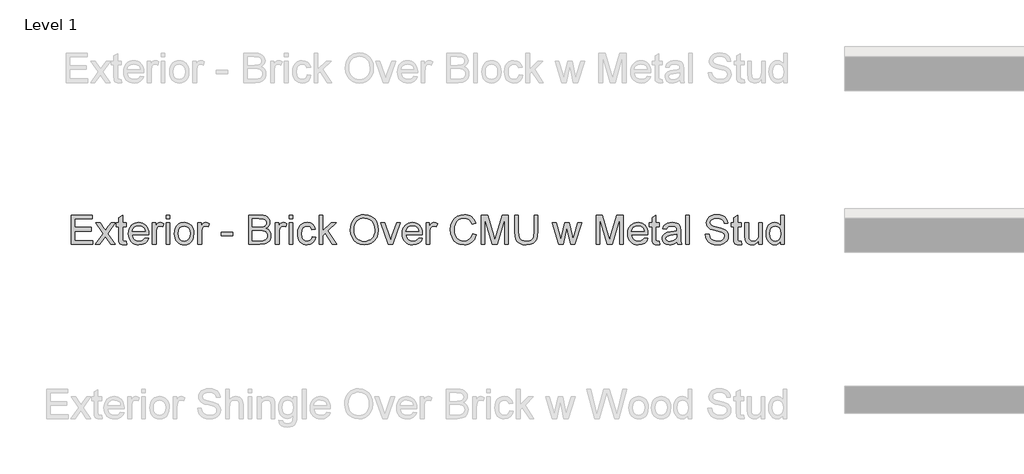
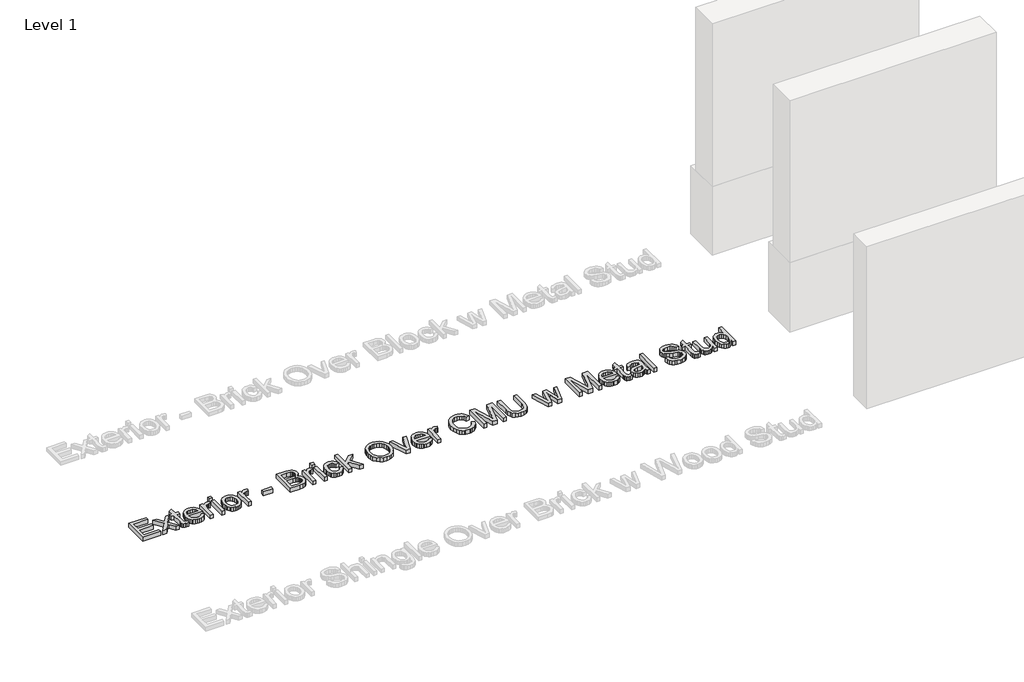
# One storey, part 39 of 42: 1 proxy.
"""IFC4 building model written with IfcOpenShell, lengths in millimetres."""

from ifc_helpers import new_model, si_unit, origin, origin_with_axes, place, context, project, spatial, polyline, outline, extrude, element, save

model = new_model("IFC4")

# Units and contexts
model_context = context("Model", 3, world=origin())
ifc_project = project(units=[si_unit("LENGTHUNIT", "METRE", prefix="MILLI")], contexts=[model_context])

# Site, building, storey
site = spatial("IfcSite", under=ifc_project)
building = spatial("IfcBuilding", under=site)
storey = spatial("IfcBuildingStorey", under=building, Name="Level 1", Elevation=0.0)

# Proxy
placement = place(None, origin())
element("IfcBuildingElementProxy", 1, Name="8\" Arial", ObjectType="8\" Arial", at=placement, inside=storey, context=model_context, shape_type="SweptSolid", body=[
    extrude(outline(polyline([(27482.7881133, 15014.0462247), (27482.7881133, 15318.6133187), (27701.6957121, 15318.6133187), (27701.6957121, 15280.542432), (27520.859, 15280.542432), (27520.859, 15190.1240759), (27692.1779905, 15190.1240759), (27692.1779905, 15152.0531892), (27520.859, 15152.0531892), (27520.859, 15052.1171114), (27706.454573, 15052.1171114), (27706.454573, 15014.0462247), (27482.7881133, 15014.0462247)])), origin_with_axes(), (0.0, 0.0, 1.0), 50.8),
    extrude(outline(polyline([(27735.0077381, 15014.0462247), (27816.3545156, 15126.4743121), (27739.7665989, 15237.7126844), (27785.5706345, 15237.7126844), (27822.5261633, 15184.1754999), (27839.7770338, 15158.8940516), (27854.7228312, 15179.5653534), (27896.8090068, 15237.7126844), (27942.6130424, 15237.7126844), (27862.1585513, 15126.4743121), (27939.6387544, 15014.0462247), (27893.8347188, 15014.0462247), (27847.2127539, 15081.6369201), (27838.6616758, 15093.9802154), (27780.8117737, 15014.0462247), (27735.0077381, 15014.0462247)])), origin_with_axes(), (0.0, 0.0, 1.0), 50.8),
    extrude(outline(polyline([(28053.8514147, 15045.7967494), (28058.6102755, 15012.9308667), (28030.1314676, 15009.2873638), (28011.8581856, 15010.8674543), (27998.2322285, 15015.6077259), (27988.602971, 15022.9133208), (27982.3197876, 15032.1893816), (27978.8621778, 15048.1204119), (27977.7096411, 15075.3909152), (27977.7096411, 15199.6417976), (27949.1564761, 15199.6417976), (27949.1564761, 15237.7126844), (27977.7096411, 15237.7126844), (27977.7096411, 15292.0677981), (28015.7805279, 15314.4493155), (28015.7805279, 15237.7126844), (28053.8514147, 15237.7126844), (28053.8514147, 15199.6417976), (28015.7805279, 15199.6417976), (28015.7805279, 15076.5062732), (28017.7881723, 15056.8759723), (28024.2944274, 15049.923574), (28037.2697589, 15047.3582506), (28053.8514147, 15045.7967494)])), origin_with_axes(), (0.0, 0.0, 1.0), 50.8),
    extrude(outline(polyline([(28248.5185661, 15080.6702765), (28285.8458808, 15075.9114156), (28272.3965222, 15047.7858045), (28250.9351751, 15026.761306), (28221.9451615, 15013.6558494), (28185.9098031, 15009.2873638), (28162.2874499, 15011.1718541), (28141.2397148, 15016.825325), (28122.7665977, 15026.2477766), (28106.8680988, 15039.4392087), (28094.0833076, 15056.0324828), (28084.9513139, 15075.6604601), (28079.4721176, 15098.3231407), (28077.6457189, 15124.0205245), (28079.4907069, 15150.5892818), (28085.0256711, 15174.0071527), (28094.2506113, 15194.2741372), (28107.1655276, 15211.3902353), (28123.0222006, 15224.9883084), (28141.0724111, 15234.7012177), (28161.316159, 15240.5289633), (28183.7534443, 15242.4715452), (28205.4680706, 15240.5336107), (28225.1053425, 15234.719807), (28242.6652602, 15225.0301343), (28258.1478236, 15211.4645925), (28270.786224, 15194.385673), (28279.8136529, 15174.1558671), (28285.2301103, 15150.7751748), (28287.0355961, 15124.2435961), (28286.8125245, 15113.9823024), (28115.7166056, 15113.9823024), (28122.3065126, 15085.4849052), (28137.6148013, 15064.5347639), (28159.7081845, 15051.6523789), (28186.6533751, 15047.3582506), (28206.9157123, 15049.3473057), (28223.9806899, 15055.3144711), (28237.8483078, 15065.6315326), (28248.5185661, 15080.6702765)]), holes=[polyline([(28115.7166056, 15152.0531892), (28248.9647093, 15152.0531892), (28243.8154732, 15172.166812), (28233.7214832, 15186.5549303), (28211.5258587, 15199.9392264), (28183.6047299, 15204.4006585), (28157.942201, 15200.8408075), (28136.7225148, 15190.1612545), (28121.9719052, 15173.5145362), (28115.7166056, 15152.0531892)])]), origin_with_axes(), (0.0, 0.0, 1.0), 50.8),
    extrude(outline(polyline([(28325.1064828, 15014.0462247), (28325.1064828, 15237.7126844), (28358.4185087, 15237.7126844), (28358.4185087, 15204.6237301), (28370.7246254, 15223.8078878), (28382.0640986, 15235.1101823), (28393.4407503, 15240.6312045), (28405.8584028, 15242.4715452), (28424.819489, 15239.5344358), (28444.0780039, 15230.7231075), (28431.3629226, 15196.5931524), (28417.9786265, 15202.4487819), (28404.5943304, 15204.4006585), (28393.2269733, 15202.5231391), (28383.0679208, 15196.8905812), (28374.8607447, 15187.9305385), (28369.3490172, 15176.070565), (28364.7202815, 15154.8044056), (28363.1773696, 15131.604959), (28363.1773696, 15014.0462247), (28325.1064828, 15014.0462247)])), origin_with_axes(), (0.0, 0.0, 1.0), 50.8),
    extrude(outline(polyline([(28467.8723082, 15280.542432), (28467.8723082, 15318.6133187), (28505.9431949, 15318.6133187), (28505.9431949, 15280.542432), (28467.8723082, 15280.542432)])), origin_with_axes(), (0.0, 0.0, 1.0), 50.8),
    extrude(outline(polyline([(28467.8723082, 15014.0462247), (28467.8723082, 15237.7126844), (28505.9431949, 15237.7126844), (28505.9431949, 15014.0462247), (28467.8723082, 15014.0462247)])), origin_with_axes(), (0.0, 0.0, 1.0), 50.8),
    extrude(outline(polyline([(28553.5318034, 15125.8794545), (28555.5905684, 15154.8462315), (28561.7668633, 15179.8070143), (28572.0606883, 15200.7618029), (28586.4720433, 15217.7105974), (28600.9809921, 15228.5435121), (28616.9956742, 15236.2813083), (28634.5160896, 15240.923986), (28653.5422383, 15242.4715452), (28674.5458238, 15240.5870549), (28693.5371176, 15234.933584), (28710.5161197, 15225.5111325), (28725.48283, 15212.3197003), (28737.6983239, 15195.8054308), (28746.4236766, 15176.414467), (28751.6588883, 15154.1468091), (28753.4039589, 15129.0024569), (28750.318135, 15090.5411949), (28741.0606635, 15061.2630471), (28725.9010892, 15039.3369675), (28705.108957, 15022.9319101), (28680.4130717, 15012.6985004), (28653.5422383, 15009.2873638), (28632.2319293, 15011.1648831), (28613.0640372, 15016.7974411), (28596.0385619, 15026.1850377), (28581.1555034, 15039.3276729), (28569.0701347, 15056.0022752), (28560.4377284, 15075.9857728), (28555.2582846, 15099.278166), (28553.5318034, 15125.8794545)]), holes=[polyline([(28591.6026901, 15125.9538117), (28596.0083543, 15091.4985438), (28609.2253467, 15066.951373), (28629.1158979, 15052.2565312), (28653.5422383, 15047.3582506), (28677.8570429, 15052.2844151), (28697.7104155, 15067.0629088), (28710.927408, 15091.9353924), (28715.3330721, 15127.1435269), (28710.899524, 15160.5949726), (28697.5988797, 15184.8075361), (28677.7176232, 15199.5023779), (28653.5422383, 15204.4006585), (28629.1158979, 15199.5209672), (28609.2253467, 15184.8818933), (28596.0083543, 15160.3904903), (28591.6026901, 15125.9538117)])]), origin_with_axes(), (0.0, 0.0, 1.0), 50.8),
    extrude(outline(polyline([(28796.2337065, 15014.0462247), (28796.2337065, 15237.7126844), (28829.5457324, 15237.7126844), (28829.5457324, 15204.6237301), (28841.8518491, 15223.8078878), (28853.1913222, 15235.1101823), (28864.5679739, 15240.6312045), (28876.9856264, 15242.4715452), (28895.9467126, 15239.5344358), (28915.2052276, 15230.7231075), (28902.4901463, 15196.5931524), (28889.1058501, 15202.4487819), (28875.721554, 15204.4006585), (28864.3541969, 15202.5231391), (28854.1951444, 15196.8905812), (28845.9879684, 15187.9305385), (28840.4762409, 15176.070565), (28835.8475051, 15154.8044056), (28834.3045932, 15131.604959), (28834.3045932, 15014.0462247), (28796.2337065, 15014.0462247)])), origin_with_axes(), (0.0, 0.0, 1.0), 50.8),
    extrude(outline(polyline([(29038.9356095, 15104.4645807), (29038.9356095, 15142.5354675), (29157.9071307, 15142.5354675), (29157.9071307, 15104.4645807), (29038.9356095, 15104.4645807)])), origin_with_axes(), (0.0, 0.0, 1.0), 50.8),
    extrude(outline(polyline([(29324.4672602, 15014.0462247), (29324.4672602, 15318.6133187), (29440.6875649, 15318.6133187), (29472.6518666, 15316.3733081), (29497.6080021, 15309.653276), (29516.7363919, 15298.285919), (29531.2174568, 15282.1039332), (29540.3355085, 15263.0684898), (29543.3748591, 15243.14076), (29540.8188303, 15224.8024154), (29533.150744, 15207.5608395), (29520.3148322, 15192.4756224), (29502.2553271, 15180.6063542), (29523.82821, 15169.3412383), (29539.7685349, 15152.2019036), (29549.6115693, 15130.3222973), (29552.8925808, 15104.8363667), (29550.6525701, 15083.5980913), (29543.9325381, 15063.9027277), (29533.9036107, 15047.1537683), (29521.7369137, 15034.7547051), (29506.8375896, 15025.7760731), (29488.6107808, 15019.2884073), (29439.7952785, 15014.0462247), (29324.4672602, 15014.0462247)]), holes=[polyline([(29362.538147, 15194.8829368), (29432.0621296, 15194.8829368), (29472.6611612, 15198.1546536), (29486.8726812, 15203.7965062), (29497.0875017, 15212.2453431), (29503.2498547, 15223.3710393), (29505.3039723, 15237.0434696), (29503.3892744, 15250.3162299), (29497.6451807, 15261.8787746), (29488.3319413, 15270.9038798), (29475.7098065, 15276.5643217), (29426.7827684, 15280.542432), (29362.538147, 15280.542432), (29362.538147, 15194.8829368)]), polyline([(29362.538147, 15052.1171114), (29440.6132077, 15052.1171114), (29468.868944, 15053.6042554), (29492.774784, 15061.8950833), (29508.6128678, 15078.8113465), (29513.2694875, 15090.7642665), (29514.821694, 15104.4645807), (29512.9999426, 15120.3770217), (29507.5346884, 15134.0587466), (29497.9890827, 15144.7568888), (29483.9262771, 15151.7185818), (29464.007842, 15155.5386829), (29436.8953477, 15156.81205), (29362.538147, 15156.81205), (29362.538147, 15052.1171114)])]), origin_with_axes(), (0.0, 0.0, 1.0), 50.8),
    extrude(outline(polyline([(29600.4811892, 15014.0462247), (29600.4811892, 15237.7126844), (29633.7932151, 15237.7126844), (29633.7932151, 15204.6237301), (29646.0993319, 15223.8078878), (29657.438805, 15235.1101823), (29668.8154567, 15240.6312045), (29681.2331092, 15242.4715452), (29700.1941954, 15239.5344358), (29719.4527104, 15230.7231075), (29706.737629, 15196.5931524), (29693.3533329, 15202.4487819), (29679.9690368, 15204.4006585), (29668.6016797, 15202.5231391), (29658.4426272, 15196.8905812), (29650.2354511, 15187.9305385), (29644.7237236, 15176.070565), (29640.0949879, 15154.8044056), (29638.552076, 15131.604959), (29638.552076, 15014.0462247), (29600.4811892, 15014.0462247)])), origin_with_axes(), (0.0, 0.0, 1.0), 50.8),
    extrude(outline(polyline([(29743.2470146, 15014.0462247), (29743.2470146, 15237.7126844), (29781.3179013, 15237.7126844), (29781.3179013, 15014.0462247), (29743.2470146, 15014.0462247)])), origin_with_axes(), (0.0, 0.0, 1.0), 50.8),
    extrude(outline(polyline([(29743.2470146, 15280.542432), (29743.2470146, 15318.6133187), (29781.3179013, 15318.6133187), (29781.3179013, 15280.542432), (29743.2470146, 15280.542432)])), origin_with_axes(), (0.0, 0.0, 1.0), 50.8),
    extrude(outline(polyline([(29981.1900568, 15094.946859), (30019.2609436, 15090.1879982), (30008.6464532, 15056.3275879), (29988.7001341, 15030.7394162), (29961.2995056, 15014.6503769), (29928.3220871, 15009.2873638), (29906.9699522, 15011.1579121), (29887.8252967, 15016.7695571), (29870.8881206, 15026.1222988), (29856.1584238, 15039.2161371), (29844.2357114, 15055.8047638), (29835.7194883, 15075.6418708), (29830.6097544, 15098.7274579), (29828.9065098, 15125.0615253), (29831.8157353, 15158.9405249), (29840.5434117, 15188.3023245), (29855.2289588, 15212.0129769), (29876.0117964, 15228.9385347), (29900.8749854, 15239.0882926), (29927.8015867, 15242.4715452), (29959.9703707, 15237.8242202), (29985.6886675, 15223.882245), (30004.1385479, 15201.3891918), (30014.5020827, 15171.0886325), (29976.431196, 15166.3297717), (29969.525271, 15182.9393114), (29958.7713608, 15194.8457582), (29944.7643231, 15202.0119334), (29928.0990155, 15204.4006585), (29903.4960767, 15199.6975655), (29883.9680169, 15185.5882867), (29871.2250516, 15161.3106606), (29866.9773965, 15126.1025261), (29871.1321051, 15090.4203644), (29883.5962309, 15066.0590866), (29902.771094, 15052.0334596), (29927.0580147, 15047.3582506), (29946.7719675, 15050.2767707), (29962.935364, 15059.0323311), (29974.6930964, 15073.8480033), (29981.1900568, 15094.946859)])), origin_with_axes(), (0.0, 0.0, 1.0), 50.8),
    extrude(outline(polyline([(30052.5729695, 15014.0462247), (30052.5729695, 15318.6133187), (30090.6438562, 15318.6133187), (30090.6438562, 15154.95312), (30176.0059227, 15237.7126844), (30228.6508207, 15237.7126844), (30142.2477535, 15153.9121192), (30233.4096816, 15014.0462247), (30188.9440756, 15014.0462247), (30114.9586609, 15127.4409557), (30090.6438562, 15103.8697231), (30090.6438562, 15014.0462247), (30052.5729695, 15014.0462247)])), origin_with_axes(), (0.0, 0.0, 1.0), 50.8),
    extrude(outline(polyline([(30376.1755069, 15162.3144829), (30378.7129464, 15198.0384705), (30386.3252648, 15229.6635174), (30399.0124622, 15257.1896236), (30416.7745385, 15280.6167892), (30438.5472563, 15299.3222725), (30463.2663783, 15312.683332), (30490.9319042, 15320.6999677), (30521.5438343, 15323.3721796), (30561.4922404, 15318.3530685), (30597.3138218, 15303.2957354), (30627.0567021, 15279.2597703), (30648.7690047, 15247.3047633), (30662.041765, 15208.9736263), (30666.4660185, 15165.8092713), (30661.8093988, 15122.068648), (30647.8395397, 15083.1984213), (30625.3278972, 15051.1876464), (30595.0459272, 15028.0253784), (30559.5310692, 15013.9718675), (30521.3207627, 15009.2873638), (30480.7589097, 15014.4644839), (30444.732846, 15029.9958442), (30415.0643229, 15054.4779525), (30393.5750919, 15086.5073167), (30380.5254032, 15123.3606043), (30376.1755069, 15162.3144829)]), holes=[polyline([(30414.2463937, 15161.9426969), (30416.1494733, 15136.7030745), (30421.8587121, 15114.2983205), (30431.3741101, 15094.7284347), (30444.6956674, 15077.9934173), (30460.8892715, 15064.5905318), (30479.0208102, 15055.0170422), (30499.0902834, 15049.2729485), (30521.0976911, 15047.3582506), (30543.4815322, 15049.2915378), (30563.788019, 15055.0913994), (30582.0171514, 15064.7578355), (30598.1689296, 15078.2908461), (30611.392893, 15095.3790603), (30620.8385812, 15115.7111073), (30626.5059941, 15139.2869873), (30628.3951317, 15166.1067001), (30625.1605935, 15199.8091013), (30615.4569788, 15228.9385347), (30599.5352432, 15252.7607229), (30577.6463422, 15270.5413885), (30551.2402413, 15281.6113167), (30521.7669059, 15285.3012928), (30500.5239831, 15283.523691), (30480.8146776, 15278.1908855), (30462.6389894, 15269.3028764), (30445.9969184, 15256.8596635), (30432.1060638, 15240.2617422), (30422.1840249, 15218.9096072), (30416.2308015, 15192.8032588), (30414.2463937, 15161.9426969)])]), origin_with_axes(), (0.0, 0.0, 1.0), 50.8),
    extrude(outline(polyline([(30768.930241, 15014.0462247), (30690.2603227, 15237.7126844), (30730.5619255, 15237.7126844), (30778.2248911, 15103.7210087), (30792.5758309, 15058.6605451), (30806.6293418, 15101.1928639), (30854.5897362, 15237.7126844), (30894.891339, 15237.7126844), (30817.1880643, 15014.0462247), (30768.930241, 15014.0462247)])), origin_with_axes(), (0.0, 0.0, 1.0), 50.8),
    extrude(outline(polyline([(31084.7996296, 15080.6702765), (31122.1269444, 15075.9114156), (31108.6775857, 15047.7858045), (31087.2162386, 15026.761306), (31058.226225, 15013.6558494), (31022.1908666, 15009.2873638), (30998.5685134, 15011.1718541), (30977.5207783, 15016.825325), (30959.0476612, 15026.2477766), (30943.1491623, 15039.4392087), (30930.3643711, 15056.0324828), (30921.2323774, 15075.6604601), (30915.7531811, 15098.3231407), (30913.9267824, 15124.0205245), (30915.7717704, 15150.5892818), (30921.3067346, 15174.0071527), (30930.5316748, 15194.2741372), (30943.4465911, 15211.3902353), (30959.3032641, 15224.9883084), (30977.3534746, 15234.7012177), (30997.5972225, 15240.5289633), (31020.0345078, 15242.4715452), (31041.7491341, 15240.5336107), (31061.386406, 15234.719807), (31078.9463237, 15225.0301343), (31094.4288871, 15211.4645925), (31107.0672876, 15194.385673), (31116.0947165, 15174.1558671), (31121.5111738, 15150.7751748), (31123.3166596, 15124.2435961), (31123.093588, 15113.9823024), (30951.9976692, 15113.9823024), (30958.5875761, 15085.4849052), (30973.8958648, 15064.5347639), (30995.989248, 15051.6523789), (31022.9344386, 15047.3582506), (31043.1967758, 15049.3473057), (31060.2617534, 15055.3144711), (31074.1293713, 15065.6315326), (31084.7996296, 15080.6702765)]), holes=[polyline([(30951.9976692, 15152.0531892), (31085.2457728, 15152.0531892), (31080.0965367, 15172.166812), (31070.0025467, 15186.5549303), (31047.8069223, 15199.9392264), (31019.8857934, 15204.4006585), (30994.2232645, 15200.8408075), (30973.0035784, 15190.1612545), (30958.2529687, 15173.5145362), (30951.9976692, 15152.0531892)])]), origin_with_axes(), (0.0, 0.0, 1.0), 50.8),
    extrude(outline(polyline([(31161.3875463, 15014.0462247), (31161.3875463, 15237.7126844), (31194.6995722, 15237.7126844), (31194.6995722, 15204.6237301), (31207.005689, 15223.8078878), (31218.3451621, 15235.1101823), (31229.7218138, 15240.6312045), (31242.1394663, 15242.4715452), (31261.1005525, 15239.5344358), (31280.3590675, 15230.7231075), (31267.6439861, 15196.5931524), (31254.25969, 15202.4487819), (31240.8753939, 15204.4006585), (31229.5080368, 15202.5231391), (31219.3489843, 15196.8905812), (31211.1418082, 15187.9305385), (31205.6300807, 15176.070565), (31201.001345, 15154.8044056), (31199.4584331, 15131.604959), (31199.4584331, 15014.0462247), (31161.3875463, 15014.0462247)])), origin_with_axes(), (0.0, 0.0, 1.0), 50.8),
    extrude(outline(polyline([(31642.0324917, 15122.3103089), (31680.1033784, 15112.4951584), (31672.5700645, 15088.819361), (31662.5364897, 15068.1317935), (31650.0026541, 15050.4324561), (31634.9685576, 15035.7213487), (31617.7734549, 15024.1564803), (31598.7566008, 15015.89586), (31577.9179954, 15010.9394879), (31555.2576384, 15009.2873638), (31511.0987559, 15014.2878856), (31492.4281275, 15020.5385377), (31476.0300411, 15029.2894508), (31449.149913, 15053.7715591), (31429.5567907, 15087.2137102), (31417.594576, 15126.53008), (31413.6071711, 15168.6348449), (31418.1150764, 15213.044683), (31431.6387923, 15251.3944093), (31453.4719253, 15282.4664245), (31482.9080822, 15305.0431296), (31517.8187879, 15318.7899171), (31556.0755676, 15323.3721796), (31577.8506091, 15321.8896829), (31597.8178412, 15317.4421928), (31615.9772638, 15310.0297094), (31632.328877, 15299.6522326), (31646.6031358, 15286.5839545), (31658.5304956, 15271.0990675), (31675.3445176, 15232.8794663), (31637.2736308, 15223.8078878), (31624.0752277, 15251.5710076), (31606.0436065, 15270.6157457), (31582.9556957, 15281.629906), (31554.5884236, 15285.3012928), (31521.8898446, 15281.2302361), (31495.0283059, 15269.0170659), (31474.6451382, 15249.9444439), (31461.3816726, 15225.2950319), (31454.1039615, 15197.4296709), (31451.6780579, 15168.7092021), (31454.5501047, 15133.5382462), (31463.1662454, 15103.1261511), (31477.8517925, 15078.6347481), (31498.9320589, 15061.2258685), (31524.2042125, 15050.8251551), (31551.4654212, 15047.3582506), (31583.2438299, 15052.0799328), (31609.724288, 15066.2449796), (31629.7170803, 15089.7046764), (31642.0324917, 15122.3103089)])), origin_with_axes(), (0.0, 0.0, 1.0), 50.8),
    extrude(outline(polyline([(31732.4508477, 15014.0462247), (31732.4508477, 15318.6133187), (31797.9595415, 15318.6133187), (31860.2708757, 15103.9440803), (31872.8372426, 15059.1066883), (31886.4446104, 15107.6619403), (31947.7149437, 15318.6133187), (32013.2236376, 15318.6133187), (32013.2236376, 15014.0462247), (31975.1527508, 15014.0462247), (31975.1527508, 15280.542432), (31898.6391913, 15014.0462247), (31847.035294, 15014.0462247), (31770.5217345, 15280.542432), (31770.5217345, 15014.0462247), (31732.4508477, 15014.0462247)])), origin_with_axes(), (0.0, 0.0, 1.0), 50.8),
    extrude(outline(polyline([(32279.7198449, 15318.6133187), (32317.7907316, 15318.6133187), (32317.7907316, 15142.9072535), (32315.2068189, 15101.7598375), (32307.4550807, 15070.0743754), (32292.9740159, 15045.6294457), (32270.2021232, 15026.203627), (32239.0836347, 15013.5164296), (32199.5627825, 15009.2873638), (32160.9063328, 15012.9680453), (32130.0016213, 15024.0100896), (32106.8393532, 15042.0324161), (32091.4102341, 15066.6539442), (32082.7383256, 15099.6778359), (32079.8476894, 15142.9072535), (32079.8476894, 15318.6133187), (32117.9185761, 15318.6133187), (32117.9185761, 15144.2456831), (32119.7960955, 15110.0320761), (32125.4286534, 15086.2098879), (32135.6341792, 15069.711884), (32151.2306021, 15057.4708299), (32171.5672964, 15049.8863954), (32195.9936369, 15047.3582506), (32234.7151491, 15052.3587723), (32249.2101559, 15058.6094245), (32260.4613299, 15067.3603376), (32268.8869302, 15079.6664543), (32274.9052161, 15096.5827174), (32279.7198449, 15144.2456831), (32279.7198449, 15318.6133187)])), origin_with_axes(), (0.0, 0.0, 1.0), 50.8),
    extrude(outline(polyline([(32535.7316869, 15014.0462247), (32467.6948482, 15237.7126844), (32507.252879, 15237.7126844), (32545.8442662, 15107.2157971), (32557.3696323, 15060.5938323), (32566.8129968, 15105.5055815), (32597.5225207, 15237.7126844), (32642.8804131, 15237.7126844), (32673.4412226, 15105.8773675), (32681.8435862, 15065.2039787), (32693.8894528, 15108.1080835), (32732.5551971, 15237.7126844), (32772.2619423, 15237.7126844), (32703.7046033, 15014.0462247), (32657.677496, 15014.0462247), (32628.4551161, 15145.2123267), (32619.9783953, 15186.1087871), (32582.2792945, 15014.0462247), (32535.7316869, 15014.0462247)])), origin_with_axes(), (0.0, 0.0, 1.0), 50.8),
    extrude(outline(polyline([(32922.1660589, 15014.0462247), (32922.1660589, 15318.6133187), (32987.6747527, 15318.6133187), (33049.9860869, 15103.9440803), (33062.5524538, 15059.1066883), (33076.1598216, 15107.6619403), (33137.4301549, 15318.6133187), (33202.9388488, 15318.6133187), (33202.9388488, 15014.0462247), (33164.867962, 15014.0462247), (33164.867962, 15280.542432), (33088.3544025, 15014.0462247), (33036.7505052, 15014.0462247), (32960.2369457, 15280.542432), (32960.2369457, 15014.0462247), (32922.1660589, 15014.0462247)])), origin_with_axes(), (0.0, 0.0, 1.0), 50.8),
    extrude(outline(polyline([(33421.4003044, 15080.6702765), (33458.7276192, 15075.9114156), (33445.2782605, 15047.7858045), (33423.8169134, 15026.761306), (33394.8268998, 15013.6558494), (33358.7915414, 15009.2873638), (33335.1691882, 15011.1718541), (33314.1214531, 15016.825325), (33295.6483361, 15026.2477766), (33279.7498371, 15039.4392087), (33266.9650459, 15056.0324828), (33257.8330522, 15075.6604601), (33252.3538559, 15098.3231407), (33250.5274572, 15124.0205245), (33252.3724452, 15150.5892818), (33257.9074094, 15174.0071527), (33267.1323496, 15194.2741372), (33280.0472659, 15211.3902353), (33295.9039389, 15224.9883084), (33313.9541494, 15234.7012177), (33334.1978973, 15240.5289633), (33356.6351826, 15242.4715452), (33378.3498089, 15240.5336107), (33397.9870808, 15234.719807), (33415.5469985, 15225.0301343), (33431.0295619, 15211.4645925), (33443.6679624, 15194.385673), (33452.6953913, 15174.1558671), (33458.1118486, 15150.7751748), (33459.9173344, 15124.2435961), (33459.6942628, 15113.9823024), (33288.598344, 15113.9823024), (33295.1882509, 15085.4849052), (33310.4965396, 15064.5347639), (33332.5899228, 15051.6523789), (33359.5351134, 15047.3582506), (33379.7974506, 15049.3473057), (33396.8624282, 15055.3144711), (33410.7300461, 15065.6315326), (33421.4003044, 15080.6702765)]), holes=[polyline([(33288.598344, 15152.0531892), (33421.8464476, 15152.0531892), (33416.6972115, 15172.166812), (33406.6032215, 15186.5549303), (33384.4075971, 15199.9392264), (33356.4864682, 15204.4006585), (33330.8239393, 15200.8408075), (33309.6042532, 15190.1612545), (33294.8536435, 15173.5145362), (33288.598344, 15152.0531892)])]), origin_with_axes(), (0.0, 0.0, 1.0), 50.8),
    extrude(outline(polyline([(33578.8888555, 15045.7967494), (33583.6477163, 15012.9308667), (33555.1689085, 15009.2873638), (33536.8956264, 15010.8674543), (33523.2696694, 15015.6077259), (33513.6404119, 15022.9133208), (33507.3572284, 15032.1893816), (33503.8996186, 15048.1204119), (33502.747082, 15075.3909152), (33502.747082, 15199.6417976), (33474.1939169, 15199.6417976), (33474.1939169, 15237.7126844), (33502.747082, 15237.7126844), (33502.747082, 15292.0677981), (33540.8179687, 15314.4493155), (33540.8179687, 15237.7126844), (33578.8888555, 15237.7126844), (33578.8888555, 15199.6417976), (33540.8179687, 15199.6417976), (33540.8179687, 15076.5062732), (33542.8256132, 15056.8759723), (33549.3318682, 15049.923574), (33562.3071997, 15047.3582506), (33578.8888555, 15045.7967494)])), origin_with_axes(), (0.0, 0.0, 1.0), 50.8),
    extrude(outline(polyline([(33759.7255676, 15042.5993897), (33741.5359374, 15027.0029669), (33722.8072175, 15016.7974411), (33703.1118539, 15011.1648831), (33682.0222929, 15009.2873638), (33650.2067056, 15013.8045638), (33626.7377141, 15027.3561636), (33612.265944, 15047.9345189), (33607.4420206, 15073.5319852), (33609.263772, 15089.3143011), (33614.7290262, 15103.6466515), (33623.1592739, 15115.9155896), (33633.8760054, 15125.5076685), (33660.5330619, 15137.9996782), (33693.4733018, 15143.7251827), (33732.3992963, 15149.7481159), (33759.502496, 15156.81205), (33759.7255676, 15165.2887709), (33757.1044763, 15182.2793912), (33749.2412023, 15193.3957928), (33731.6557243, 15201.649442), (33707.1550267, 15204.4006585), (33684.4760805, 15202.5696124), (33668.6379967, 15197.0764742), (33657.8376133, 15186.9174216), (33650.2717682, 15171.0886325), (33612.2008814, 15175.8474934), (33618.8093776, 15196.6675096), (33628.6710014, 15213.0260937), (33642.705923, 15225.5366928), (33661.8343129, 15234.8127535), (33685.2289471, 15240.5568473), (33712.062602, 15242.4715452), (33737.799488, 15240.7799189), (33758.201245, 15235.7050399), (33773.5838909, 15228.0741322), (33784.2634438, 15218.7144196), (33791.3459672, 15207.1425802), (33795.9375243, 15192.8752923), (33797.7964544, 15159.5632664), (33797.7964544, 15112.1977296), (33799.7297416, 15046.0569996), (33807.314176, 15014.0462247), (33769.2432893, 15014.0462247), (33763.1459988, 15027.2818064), (33759.7255676, 15042.5993897)]), holes=[polyline([(33759.7255676, 15118.7411632), (33698.3065198, 15107.0670827), (33665.5521729, 15100.8954351), (33650.7179114, 15090.857213), (33645.5129073, 15076.2088444), (33648.3477756, 15064.8879606), (33656.8523804, 15055.6118999), (33670.8408288, 15049.4216629), (33690.1272277, 15047.3582506), (33710.5754579, 15049.6354398), (33728.6442577, 15056.4670077), (33743.2926262, 15066.5331137), (33753.4795627, 15078.5139177), (33757.9967627, 15090.857213), (33759.502496, 15107.9593691), (33759.7255676, 15118.7411632)])]), origin_with_axes(), (0.0, 0.0, 1.0), 50.8),
    extrude(outline(polyline([(33850.1439237, 15014.0462247), (33850.1439237, 15318.6133187), (33888.2148104, 15318.6133187), (33888.2148104, 15014.0462247), (33850.1439237, 15014.0462247)])), origin_with_axes(), (0.0, 0.0, 1.0), 50.8),
    extrude(outline(polyline([(34054.77494, 15118.7411632), (34092.8458267, 15118.7411632), (34097.2143123, 15097.6144236), (34105.1147649, 15080.6330979), (34117.4394709, 15067.1558553), (34135.0807167, 15056.5413649), (34156.6443049, 15049.6540291), (34180.736038, 15047.3582506), (34201.9464295, 15049.0963501), (34220.5171403, 15054.3106488), (34235.5651788, 15062.5642981), (34246.2075532, 15073.4204494), (34252.5372099, 15085.8845752), (34254.6470955, 15098.9621479), (34253.0670049, 15111.7051131), (34248.3267334, 15122.7192735), (34238.6974759, 15132.1161647), (34222.4504276, 15140.0073226), (34167.0171344, 15154.5441554), (34130.6285793, 15164.1641182), (34107.3454809, 15173.3193486), (34088.3936893, 15186.1273764), (34074.96292, 15201.649442), (34066.9602262, 15219.5509381), (34064.2926617, 15239.4972572), (34067.5922624, 15261.7951227), (34077.4910648, 15282.587255), (34093.7288185, 15300.2099116), (34116.0452734, 15312.9993501), (34142.8324549, 15320.7789722), (34172.4823887, 15323.3721796), (34204.6046994, 15320.6581417), (34232.7117213, 15312.5160283), (34255.7996321, 15299.1131428), (34272.8646096, 15280.6167892), (34283.664993, 15258.1795039), (34287.9591214, 15232.9538235), (34249.8882346, 15232.9538235), (34242.8986578, 15255.6699483), (34228.3246464, 15272.0657111), (34205.5527537, 15281.9923974), (34173.9695327, 15285.3012928), (34141.6427397, 15282.029576), (34119.4657046, 15272.2144255), (34106.6390875, 15257.7705393), (34102.3635484, 15240.6126152), (34105.3936044, 15225.982836), (34114.4837721, 15214.2158089), (34135.9730031, 15203.694265), (34176.6463919, 15192.9496495), (34218.6210317, 15182.7441238), (34244.0140158, 15173.839849), (34265.7170237, 15160.0279989), (34280.8580087, 15142.9816107), (34289.7529888, 15122.8865772), (34292.7179822, 15099.9287915), (34289.3068456, 15076.4598), (34279.0734359, 15054.385006), (34262.4360122, 15035.3867413), (34239.8128339, 15021.1473373), (34212.6073931, 15012.2523572), (34182.223182, 15009.2873638), (34144.9237512, 15012.4847234), (34114.2235219, 15022.0768023), (34089.7692976, 15038.1007791), (34071.2078813, 15060.5938323), (34059.2921399, 15087.9944608), (34054.77494, 15118.7411632)])), origin_with_axes(), (0.0, 0.0, 1.0), 50.8),
    extrude(outline(polyline([(34425.9660859, 15045.7967494), (34430.7249467, 15012.9308667), (34402.2461389, 15009.2873638), (34383.9728568, 15010.8674543), (34370.3468998, 15015.6077259), (34360.7176423, 15022.9133208), (34354.4344588, 15032.1893816), (34350.976849, 15048.1204119), (34349.8243124, 15075.3909152), (34349.8243124, 15199.6417976), (34321.2711473, 15199.6417976), (34321.2711473, 15237.7126844), (34349.8243124, 15237.7126844), (34349.8243124, 15292.0677981), (34387.8951991, 15314.4493155), (34387.8951991, 15237.7126844), (34425.9660859, 15237.7126844), (34425.9660859, 15199.6417976), (34387.8951991, 15199.6417976), (34387.8951991, 15076.5062732), (34389.9028435, 15056.8759723), (34396.4090986, 15049.923574), (34409.3844301, 15047.3582506), (34425.9660859, 15045.7967494)])), origin_with_axes(), (0.0, 0.0, 1.0), 50.8),
    extrude(outline(polyline([(34606.802798, 15014.0462247), (34606.802798, 15052.4888974), (34593.0281265, 15033.5882265), (34576.9855605, 15020.0877472), (34558.6750998, 15011.9874597), (34538.0967445, 15009.2873638), (34519.5539176, 15011.1834724), (34502.2937524, 15016.8717983), (34487.8126876, 15025.4228764), (34477.6071618, 15035.9072417), (34470.7384153, 15048.6409123), (34466.2676887, 15063.9399063), (34464.0369726, 15099.3339339), (34464.0369726, 15237.7126844), (34502.1078594, 15237.7126844), (34502.1078594, 15117.2540192), (34504.4129326, 15078.4395605), (34509.9618387, 15065.4921129), (34519.4702658, 15055.6490785), (34532.3061775, 15049.4309575), (34547.8375378, 15047.3582506), (34564.2611845, 15049.4774308), (34579.6252411, 15055.8349715), (34592.2938492, 15065.8453096), (34600.6311503, 15078.9228823), (34605.2598861, 15096.833673), (34606.802798, 15121.3436653), (34606.802798, 15237.7126844), (34644.8736847, 15237.7126844), (34644.8736847, 15014.0462247), (34606.802798, 15014.0462247)])), origin_with_axes(), (0.0, 0.0, 1.0), 50.8),
    extrude(outline(polyline([(34835.2281185, 15014.0462247), (34835.2281185, 15049.9607526), (34823.8375248, 15032.166145), (34810.0396168, 15019.455711), (34793.8343944, 15011.8294506), (34775.2218576, 15009.2873638), (34750.6096241, 15012.9680453), (34728.0793923, 15024.0100896), (34709.0067703, 15041.6420408), (34694.7673664, 15065.0924429), (34685.9002702, 15093.4132418), (34682.9445715, 15125.6563829), (34685.667904, 15157.4998541), (34693.8379014, 15186.2575015), (34707.4452691, 15210.2934666), (34726.4807125, 15227.9718911), (34749.5035608, 15238.8466317), (34775.0731432, 15242.4715452), (34793.6996219, 15239.8783378), (34810.1697419, 15232.0987157), (34824.1303063, 15220.1736797), (34835.2281185, 15205.1442305), (34835.2281185, 15318.6133187), (34873.2990053, 15318.6133187), (34873.2990053, 15014.0462247), (34835.2281185, 15014.0462247)]), holes=[polyline([(34721.0154583, 15125.8050973), (34725.3095866, 15091.3684187), (34738.1919716, 15066.8770158), (34756.9113969, 15052.2379419), (34778.716646, 15047.3582506), (34800.5126005, 15052.0148703), (34818.7579986, 15065.9847294), (34831.1105885, 15089.528078), (34835.2281185, 15122.9051665), (34831.0362313, 15159.3959627), (34818.4605698, 15184.6960003), (34799.7504391, 15199.4744939), (34777.1551448, 15204.4006585), (34755.1268241, 15199.6696816), (34737.0766136, 15185.4767509), (34725.0307471, 15161.0968837), (34721.0154583, 15125.8050973)])]), origin_with_axes(), (0.0, 0.0, 1.0), 50.8),
])

save(model, "model.ifc")

# Revit data of these elements
# Element 1 (IfcBuildingElementProxy, "8\" Arial")
#   Phase Created = New Construction
